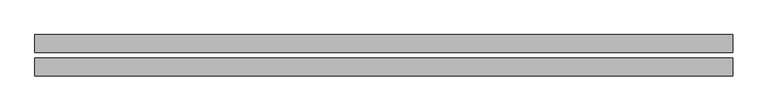
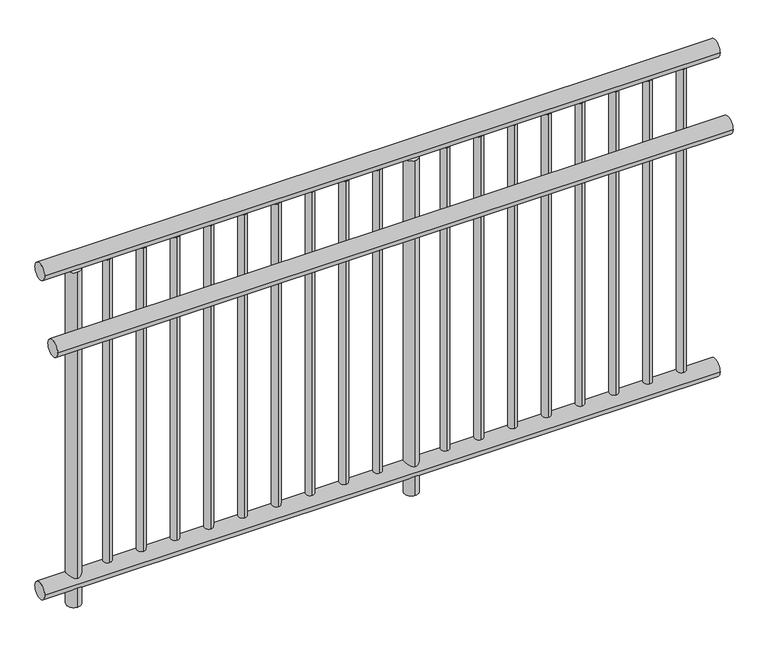
"""IFC4 building model written with IfcOpenShell, lengths in millimetres: railing geometry."""

import ifcopenshell
import ifcopenshell.guid

model = None  # the IFC model being written
_history = None  # IfcOwnerHistory: only IFC2X3 demands one
_inside = {}  # id of a spatial element -> (the spatial element, [elements in it])
_under = {}  # id of a project, library or spatial element -> (it, [spatial elements below it])
_declared = {}  # id of a project -> (the project, [libraries it declares])
_typed = {}  # id of a type object -> (the type object, [elements of that type])
_made_of = {}  # id of a material, layer set ... -> (it, [elements and type objects made of it])


def new_model(schema):
    """Start an empty IFC model of exactly this schema.

    Asked for "IFC4X3", IfcOpenShell would pick the latest addendum, in which some entities
    have other attributes; the version numbers below select the first issue.
    IFC2X3 requires an IfcOwnerHistory on every rooted entity: one is made here for all.
    """
    global model, _history
    if schema == "IFC4X3":
        model = ifcopenshell.file(schema_version=(4, 3, 0, 0))
    else:
        model = ifcopenshell.file(schema=schema)
    _inside.clear()
    _under.clear()
    _declared.clear()
    _typed.clear()
    _made_of.clear()
    _history = None
    if model.schema == "IFC2X3":
        org = make("IfcOrganization", Name="unknown")
        user = make(
            "IfcPersonAndOrganization",
            ThePerson=make("IfcPerson", FamilyName="unknown"),
            TheOrganization=org,
        )
        app = make(
            "IfcApplication",
            ApplicationDeveloper=org,
            Version="unknown",
            ApplicationFullName="unknown",
            ApplicationIdentifier="unknown",
        )
        _history = make(
            "IfcOwnerHistory",
            OwningUser=user,
            OwningApplication=app,
            ChangeAction="ADDED",
            CreationDate=0,
        )
    return model


def make(cls, **values):
    """One entity of the class cls with the attributes given. An attribute that is None is left unset."""
    return model.create_entity(
        cls, **{name: value for name, value in values.items() if value is not None}
    )


def rooted(cls, **values):
    """An entity with a GlobalId (a new one), such as an element, a storey or a relation."""
    return make(cls, GlobalId=ifcopenshell.guid.new(), OwnerHistory=_history, **values)


def si_unit(unit_type, name, prefix=None):
    """IfcSIUnit, for example si_unit("LENGTHUNIT", "METRE", prefix="MILLI")."""
    return make("IfcSIUnit", UnitType=unit_type, Prefix=prefix, Name=name)


def assignment(units):
    """IfcUnitAssignment: the units of a project."""
    return None if units is None else make("IfcUnitAssignment", Units=units)


def point(xyz):
    """IfcCartesianPoint."""
    return None if xyz is None else make("IfcCartesianPoint", Coordinates=xyz)


def direction(xyz):
    """IfcDirection."""
    return None if xyz is None else make("IfcDirection", DirectionRatios=xyz)


def frame(location, z_axis=None, x_axis=None):
    """IfcAxis2Placement3D, a coordinate frame: its origin and axes. An axis left out is left unset."""
    return make(
        "IfcAxis2Placement3D",
        Location=point(location),
        Axis=direction(z_axis),
        RefDirection=direction(x_axis),
    )


def frame_2d(location, x_axis=None):
    """IfcAxis2Placement2D, a coordinate frame in the plane: its origin and x axis."""
    return make(
        "IfcAxis2Placement2D", Location=point(location), RefDirection=direction(x_axis)
    )


def origin():
    """The frame at (0, 0, 0) with its axes left unset."""
    return frame((0.0, 0.0, 0.0))


def origin_with_axes():
    """The frame at (0, 0, 0) with the z axis (0, 0, 1) and the x axis (1, 0, 0) written out."""
    return frame((0.0, 0.0, 0.0), z_axis=(0.0, 0.0, 1.0), x_axis=(1.0, 0.0, 0.0))


def place(relative_to, where):
    """IfcLocalPlacement: puts the frame where relative to a parent placement (None: the world)."""
    return make(
        "IfcLocalPlacement", PlacementRelTo=relative_to, RelativePlacement=where
    )


def context(
    kind, dimensions, precision=None, world=None, true_north=None, identifier=None
):
    """IfcGeometricRepresentationContext, for example the 3D "Model" context."""
    return make(
        "IfcGeometricRepresentationContext",
        ContextIdentifier=identifier,
        ContextType=kind,
        CoordinateSpaceDimension=dimensions,
        Precision=precision,
        WorldCoordinateSystem=world,
        TrueNorth=true_north,
    )


def project(units=None, contexts=None):
    """IfcProject with its units and contexts."""
    return rooted(
        "IfcProject",
        Name="project",
        RepresentationContexts=contexts,
        UnitsInContext=assignment(units),
    )


def spatial(cls, under=None, at=None, **own):
    """A site, building, storey or space (cls), placed at a placement, below another one or the project."""
    s = rooted(cls, ObjectPlacement=at, **own)
    if under is not None:
        _under.setdefault(under.id(), (under, []))[1].append(s)
    return s


def circle_curve(where, radius):
    """IfcCircle in the frame where."""
    return make("IfcCircle", Position=where, Radius=radius)


def trimmed(basis, trim1, trim2, sense, master):
    """IfcTrimmedCurve: the piece of a basis curve between two trims."""
    return make(
        "IfcTrimmedCurve",
        BasisCurve=basis,
        Trim1=trim1,
        Trim2=trim2,
        SenseAgreement=sense,
        MasterRepresentation=master,
    )


def segment(curve, same_sense, transition):
    """IfcCompositeCurveSegment."""
    return make(
        "IfcCompositeCurveSegment",
        Transition=transition,
        SameSense=same_sense,
        ParentCurve=curve,
    )


def composite_curve(segments, self_intersect=None):
    """IfcCompositeCurve: segments joined end to end."""
    return make("IfcCompositeCurve", Segments=segments, SelfIntersect=self_intersect)


def outline(outer, holes=None, kind="AREA"):
    """IfcArbitraryClosedProfileDef: a profile drawn as a closed curve; with holes, ...WithVoids."""
    if holes is None:
        return make("IfcArbitraryClosedProfileDef", ProfileType=kind, OuterCurve=outer)
    return make(
        "IfcArbitraryProfileDefWithVoids",
        ProfileType=kind,
        OuterCurve=outer,
        InnerCurves=holes,
    )


def extrude(swept, where, along, depth):
    """IfcExtrudedAreaSolid: the profile swept, set in the frame where, extruded along a direction by depth."""
    return make(
        "IfcExtrudedAreaSolid",
        SweptArea=swept,
        Position=where,
        ExtrudedDirection=direction(along),
        Depth=depth,
    )


def shape(context_of_items, identifier, shape_type, items):
    """IfcShapeRepresentation: the items that make up one representation, for example the "Body"."""
    return make(
        "IfcShapeRepresentation",
        ContextOfItems=context_of_items,
        RepresentationIdentifier=identifier,
        RepresentationType=shape_type,
        Items=items,
    )


def source(mapping_origin, context_of_items, identifier, shape_type, items):
    """IfcRepresentationMap: a shape defined once, which mapped items show again and again."""
    return make(
        "IfcRepresentationMap",
        MappingOrigin=mapping_origin,
        MappedRepresentation=shape(context_of_items, identifier, shape_type, items),
    )


def transform(
    local_origin,
    x_axis=None,
    y_axis=None,
    z_axis=None,
    scale=None,
    scale2=None,
    scale3=None,
    uniform=True,
):
    """IfcCartesianTransformationOperator3D, or its non-uniform kind. x_axis, y_axis, z_axis: its Axis1, 2, 3."""
    if uniform:
        return make(
            "IfcCartesianTransformationOperator3D",
            Axis1=direction(x_axis),
            Axis2=direction(y_axis),
            LocalOrigin=point(local_origin),
            Scale=scale,
            Axis3=direction(z_axis),
        )
    return make(
        "IfcCartesianTransformationOperator3DnonUniform",
        Axis1=direction(x_axis),
        Axis2=direction(y_axis),
        LocalOrigin=point(local_origin),
        Scale=scale,
        Axis3=direction(z_axis),
        Scale2=scale2,
        Scale3=scale3,
    )


def mapped(mapping_source, mapping_target):
    """IfcMappedItem: shows the shape of a source again, moved by a transform."""
    return make(
        "IfcMappedItem", MappingSource=mapping_source, MappingTarget=mapping_target
    )


def made_of(thing, what):
    """Note that an element or type object is made of a material, layer set ...; save() writes the relation."""
    if what is not None:
        _made_of.setdefault(what.id(), (what, []))[1].append(thing)
    return thing


def element(
    cls,
    number,
    at=None,
    inside=None,
    cuts=None,
    type_object=None,
    material=None,
    context=None,
    identifier="Body",
    shape_type=None,
    held_by="IfcProductDefinitionShape",
    body=None,
    shapes=None,
    **own,
):
    """One element of the class cls, such as IfcWall. Its Tag is "e" and its number.

    at: its placement. inside: the storey or other place that contains it. cuts: it is an
    opening in that element (IfcRelVoidsElement). A single representation is given by context,
    identifier, shape_type and body (its items); several are given by shapes. held_by: the class
    of the entity that holds the representations. save() writes the other relations.
    """
    e = rooted(cls, Tag="e%d" % number, ObjectPlacement=at, **own)
    if body is not None:
        shapes = [shape(context, identifier, shape_type, body)]
    if shapes is not None:
        e.Representation = make(held_by, Representations=shapes)
    if inside is not None:
        _inside.setdefault(inside.id(), (inside, []))[1].append(e)
    if cuts is not None:
        rooted(
            "IfcRelVoidsElement", RelatingBuildingElement=cuts, RelatedOpeningElement=e
        )
    if type_object is not None:
        _typed.setdefault(type_object.id(), (type_object, []))[1].append(e)
    return made_of(e, material)


def aggregate(whole, parts):
    """IfcRelAggregates: a whole, such as a stair, and the parts it consists of."""
    return rooted("IfcRelAggregates", RelatingObject=whole, RelatedObjects=parts)


def save(model, path):
    """Write the relations noted so far, then the file.

    IfcRelAggregates (storeys below a building ...), IfcRelContainedInSpatialStructure (elements
    in a storey), IfcRelDefinesByType, IfcRelAssociatesMaterial and IfcRelDeclares: one each for
    every whole, place, type object, material and project.
    """
    for whole, parts in _under.values():
        aggregate(whole, parts)
    for where, things in _inside.values():
        rooted(
            "IfcRelContainedInSpatialStructure",
            RelatedElements=things,
            RelatingStructure=where,
        )
    for kind, things in _typed.values():
        rooted("IfcRelDefinesByType", RelatedObjects=things, RelatingType=kind)
    for what, things in _made_of.values():
        rooted("IfcRelAssociatesMaterial", RelatedObjects=things, RelatingMaterial=what)
    for by, libraries in _declared.values():
        rooted("IfcRelDeclares", RelatingContext=by, RelatedDefinitions=libraries)
    model.write(path)


def railing_eefe8ac2(model_context):
    return source(origin(), model_context, "Body", "SweptSolid", [
        extrude(outline(composite_curve([segment(trimmed(circle_curve(frame_2d((29848.1400611, 1074.6)), 25.4), [point((29873.5400611, 1074.6))], [point((29822.7400611, 1074.6))], False, "CARTESIAN"), True, "CONTINUOUS"), segment(trimmed(circle_curve(frame_2d((29848.1400611, 1074.6)), 25.4), [point((29822.7400611, 1074.6))], [point((29873.5400611, 1074.6))], False, "CARTESIAN"), True, "CONTINUOUS")], self_intersect=False)), frame((9666.6129185, 0.0, 0.0), z_axis=(1.0, 0.0, 0.0), x_axis=(0.0, 1.0, 0.0)), (0.0, 0.0, 1.0), 2000.0),
        extrude(outline(composite_curve([segment(trimmed(circle_curve(frame_2d((29781.1400611, 874.6)), 25.4), [point((29806.5400611, 874.6))], [point((29755.7400611, 874.6))], False, "CARTESIAN"), True, "CONTINUOUS"), segment(trimmed(circle_curve(frame_2d((29781.1400611, 874.6)), 25.4), [point((29755.7400611, 874.6))], [point((29806.5400611, 874.6))], False, "CARTESIAN"), True, "CONTINUOUS")], self_intersect=False)), frame((9666.6129185, 0.0, 0.0), z_axis=(1.0, 0.0, 0.0), x_axis=(0.0, 1.0, 0.0)), (0.0, 0.0, 1.0), 2000.0),
        extrude(outline(composite_curve([segment(trimmed(circle_curve(frame_2d((29848.1400611, 74.6)), 25.4), [point((29873.5400611, 74.6))], [point((29822.7400611, 74.6))], False, "CARTESIAN"), True, "CONTINUOUS"), segment(trimmed(circle_curve(frame_2d((29848.1400611, 74.6)), 25.4), [point((29822.7400611, 74.6))], [point((29873.5400611, 74.6))], False, "CARTESIAN"), True, "CONTINUOUS")], self_intersect=False)), frame((9666.6129185, 0.0, 0.0), z_axis=(1.0, 0.0, 0.0), x_axis=(0.0, 1.0, 0.0)), (0.0, 0.0, 1.0), 2000.0),
        extrude(outline(composite_curve([segment(trimmed(circle_curve(frame_2d((11566.6129185, 29848.1400611)), 12.5), [point((11566.6129185, 29860.6400611))], [point((11566.6129185, 29835.6400611))], False, "CARTESIAN"), True, "CONTINUOUS"), segment(trimmed(circle_curve(frame_2d((11566.6129185, 29848.1400611)), 12.5), [point((11566.6129185, 29835.6400611))], [point((11566.6129185, 29860.6400611))], False, "CARTESIAN"), True, "CONTINUOUS")], self_intersect=False)), frame((0.0, 0.0, 100.0), z_axis=(0.0, 0.0, 1.0), x_axis=(1.0, 0.0, 0.0)), (0.0, 0.0, 1.0), 949.2),
        extrude(outline(composite_curve([segment(trimmed(circle_curve(frame_2d((11466.6129185, 29848.1400611)), 12.5), [point((11466.6129185, 29860.6400611))], [point((11466.6129185, 29835.6400611))], False, "CARTESIAN"), True, "CONTINUOUS"), segment(trimmed(circle_curve(frame_2d((11466.6129185, 29848.1400611)), 12.5), [point((11466.6129185, 29835.6400611))], [point((11466.6129185, 29860.6400611))], False, "CARTESIAN"), True, "CONTINUOUS")], self_intersect=False)), frame((0.0, 0.0, 100.0), z_axis=(0.0, 0.0, 1.0), x_axis=(1.0, 0.0, 0.0)), (0.0, 0.0, 1.0), 949.2),
        extrude(outline(composite_curve([segment(trimmed(circle_curve(frame_2d((11366.6129185, 29848.1400611)), 12.5), [point((11366.6129185, 29860.6400611))], [point((11366.6129185, 29835.6400611))], False, "CARTESIAN"), True, "CONTINUOUS"), segment(trimmed(circle_curve(frame_2d((11366.6129185, 29848.1400611)), 12.5), [point((11366.6129185, 29835.6400611))], [point((11366.6129185, 29860.6400611))], False, "CARTESIAN"), True, "CONTINUOUS")], self_intersect=False)), frame((0.0, 0.0, 100.0), z_axis=(0.0, 0.0, 1.0), x_axis=(1.0, 0.0, 0.0)), (0.0, 0.0, 1.0), 949.2),
        extrude(outline(composite_curve([segment(trimmed(circle_curve(frame_2d((11266.6129185, 29848.1400611)), 12.5), [point((11266.6129185, 29860.6400611))], [point((11266.6129185, 29835.6400611))], False, "CARTESIAN"), True, "CONTINUOUS"), segment(trimmed(circle_curve(frame_2d((11266.6129185, 29848.1400611)), 12.5), [point((11266.6129185, 29835.6400611))], [point((11266.6129185, 29860.6400611))], False, "CARTESIAN"), True, "CONTINUOUS")], self_intersect=False)), frame((0.0, 0.0, 100.0), z_axis=(0.0, 0.0, 1.0), x_axis=(1.0, 0.0, 0.0)), (0.0, 0.0, 1.0), 949.2),
        extrude(outline(composite_curve([segment(trimmed(circle_curve(frame_2d((11166.6129185, 29848.1400611)), 12.5), [point((11166.6129185, 29860.6400611))], [point((11166.6129185, 29835.6400611))], False, "CARTESIAN"), True, "CONTINUOUS"), segment(trimmed(circle_curve(frame_2d((11166.6129185, 29848.1400611)), 12.5), [point((11166.6129185, 29835.6400611))], [point((11166.6129185, 29860.6400611))], False, "CARTESIAN"), True, "CONTINUOUS")], self_intersect=False)), frame((0.0, 0.0, 100.0), z_axis=(0.0, 0.0, 1.0), x_axis=(1.0, 0.0, 0.0)), (0.0, 0.0, 1.0), 949.2),
        extrude(outline(composite_curve([segment(trimmed(circle_curve(frame_2d((11066.6129185, 29848.1400611)), 12.5), [point((11066.6129185, 29860.6400611))], [point((11066.6129185, 29835.6400611))], False, "CARTESIAN"), True, "CONTINUOUS"), segment(trimmed(circle_curve(frame_2d((11066.6129185, 29848.1400611)), 12.5), [point((11066.6129185, 29835.6400611))], [point((11066.6129185, 29860.6400611))], False, "CARTESIAN"), True, "CONTINUOUS")], self_intersect=False)), frame((0.0, 0.0, 100.0), z_axis=(0.0, 0.0, 1.0), x_axis=(1.0, 0.0, 0.0)), (0.0, 0.0, 1.0), 949.2),
        extrude(outline(composite_curve([segment(trimmed(circle_curve(frame_2d((10966.6129185, 29848.1400611)), 12.5), [point((10966.6129185, 29860.6400611))], [point((10966.6129185, 29835.6400611))], False, "CARTESIAN"), True, "CONTINUOUS"), segment(trimmed(circle_curve(frame_2d((10966.6129185, 29848.1400611)), 12.5), [point((10966.6129185, 29835.6400611))], [point((10966.6129185, 29860.6400611))], False, "CARTESIAN"), True, "CONTINUOUS")], self_intersect=False)), frame((0.0, 0.0, 100.0), z_axis=(0.0, 0.0, 1.0), x_axis=(1.0, 0.0, 0.0)), (0.0, 0.0, 1.0), 949.2),
        extrude(outline(composite_curve([segment(trimmed(circle_curve(frame_2d((10866.6129185, 29848.1400611)), 12.5), [point((10866.6129185, 29860.6400611))], [point((10866.6129185, 29835.6400611))], False, "CARTESIAN"), True, "CONTINUOUS"), segment(trimmed(circle_curve(frame_2d((10866.6129185, 29848.1400611)), 12.5), [point((10866.6129185, 29835.6400611))], [point((10866.6129185, 29860.6400611))], False, "CARTESIAN"), True, "CONTINUOUS")], self_intersect=False)), frame((0.0, 0.0, 100.0), z_axis=(0.0, 0.0, 1.0), x_axis=(1.0, 0.0, 0.0)), (0.0, 0.0, 1.0), 949.2),
        extrude(outline(composite_curve([segment(trimmed(circle_curve(frame_2d((10766.6129185, 29848.1400611)), 21.0), [point((10766.6129185, 29869.1400611))], [point((10766.6129185, 29827.1400611))], False, "CARTESIAN"), True, "CONTINUOUS"), segment(trimmed(circle_curve(frame_2d((10766.6129185, 29848.1400611)), 21.0), [point((10766.6129185, 29827.1400611))], [point((10766.6129185, 29869.1400611))], False, "CARTESIAN"), True, "CONTINUOUS")], self_intersect=False)), origin_with_axes(), (0.0, 0.0, 1.0), 1049.2),
        extrude(outline(composite_curve([segment(trimmed(circle_curve(frame_2d((10666.6129185, 29848.1400611)), 12.5), [point((10666.6129185, 29860.6400611))], [point((10666.6129185, 29835.6400611))], False, "CARTESIAN"), True, "CONTINUOUS"), segment(trimmed(circle_curve(frame_2d((10666.6129185, 29848.1400611)), 12.5), [point((10666.6129185, 29835.6400611))], [point((10666.6129185, 29860.6400611))], False, "CARTESIAN"), True, "CONTINUOUS")], self_intersect=False)), frame((0.0, 0.0, 100.0), z_axis=(0.0, 0.0, 1.0), x_axis=(1.0, 0.0, 0.0)), (0.0, 0.0, 1.0), 949.2),
        extrude(outline(composite_curve([segment(trimmed(circle_curve(frame_2d((10566.6129185, 29848.1400611)), 12.5), [point((10566.6129185, 29860.6400611))], [point((10566.6129185, 29835.6400611))], False, "CARTESIAN"), True, "CONTINUOUS"), segment(trimmed(circle_curve(frame_2d((10566.6129185, 29848.1400611)), 12.5), [point((10566.6129185, 29835.6400611))], [point((10566.6129185, 29860.6400611))], False, "CARTESIAN"), True, "CONTINUOUS")], self_intersect=False)), frame((0.0, 0.0, 100.0), z_axis=(0.0, 0.0, 1.0), x_axis=(1.0, 0.0, 0.0)), (0.0, 0.0, 1.0), 949.2),
        extrude(outline(composite_curve([segment(trimmed(circle_curve(frame_2d((10466.6129185, 29848.1400611)), 12.5), [point((10466.6129185, 29860.6400611))], [point((10466.6129185, 29835.6400611))], False, "CARTESIAN"), True, "CONTINUOUS"), segment(trimmed(circle_curve(frame_2d((10466.6129185, 29848.1400611)), 12.5), [point((10466.6129185, 29835.6400611))], [point((10466.6129185, 29860.6400611))], False, "CARTESIAN"), True, "CONTINUOUS")], self_intersect=False)), frame((0.0, 0.0, 100.0), z_axis=(0.0, 0.0, 1.0), x_axis=(1.0, 0.0, 0.0)), (0.0, 0.0, 1.0), 949.2),
        extrude(outline(composite_curve([segment(trimmed(circle_curve(frame_2d((10366.6129185, 29848.1400611)), 12.5), [point((10366.6129185, 29860.6400611))], [point((10366.6129185, 29835.6400611))], False, "CARTESIAN"), True, "CONTINUOUS"), segment(trimmed(circle_curve(frame_2d((10366.6129185, 29848.1400611)), 12.5), [point((10366.6129185, 29835.6400611))], [point((10366.6129185, 29860.6400611))], False, "CARTESIAN"), True, "CONTINUOUS")], self_intersect=False)), frame((0.0, 0.0, 100.0), z_axis=(0.0, 0.0, 1.0), x_axis=(1.0, 0.0, 0.0)), (0.0, 0.0, 1.0), 949.2),
        extrude(outline(composite_curve([segment(trimmed(circle_curve(frame_2d((10266.6129185, 29848.1400611)), 12.5), [point((10266.6129185, 29860.6400611))], [point((10266.6129185, 29835.6400611))], False, "CARTESIAN"), True, "CONTINUOUS"), segment(trimmed(circle_curve(frame_2d((10266.6129185, 29848.1400611)), 12.5), [point((10266.6129185, 29835.6400611))], [point((10266.6129185, 29860.6400611))], False, "CARTESIAN"), True, "CONTINUOUS")], self_intersect=False)), frame((0.0, 0.0, 100.0), z_axis=(0.0, 0.0, 1.0), x_axis=(1.0, 0.0, 0.0)), (0.0, 0.0, 1.0), 949.2),
        extrude(outline(composite_curve([segment(trimmed(circle_curve(frame_2d((10166.6129185, 29848.1400611)), 12.5), [point((10166.6129185, 29860.6400611))], [point((10166.6129185, 29835.6400611))], False, "CARTESIAN"), True, "CONTINUOUS"), segment(trimmed(circle_curve(frame_2d((10166.6129185, 29848.1400611)), 12.5), [point((10166.6129185, 29835.6400611))], [point((10166.6129185, 29860.6400611))], False, "CARTESIAN"), True, "CONTINUOUS")], self_intersect=False)), frame((0.0, 0.0, 100.0), z_axis=(0.0, 0.0, 1.0), x_axis=(1.0, 0.0, 0.0)), (0.0, 0.0, 1.0), 949.2),
        extrude(outline(composite_curve([segment(trimmed(circle_curve(frame_2d((10066.6129185, 29848.1400611)), 12.5), [point((10066.6129185, 29860.6400611))], [point((10066.6129185, 29835.6400611))], False, "CARTESIAN"), True, "CONTINUOUS"), segment(trimmed(circle_curve(frame_2d((10066.6129185, 29848.1400611)), 12.5), [point((10066.6129185, 29835.6400611))], [point((10066.6129185, 29860.6400611))], False, "CARTESIAN"), True, "CONTINUOUS")], self_intersect=False)), frame((0.0, 0.0, 100.0), z_axis=(0.0, 0.0, 1.0), x_axis=(1.0, 0.0, 0.0)), (0.0, 0.0, 1.0), 949.2),
        extrude(outline(composite_curve([segment(trimmed(circle_curve(frame_2d((9966.6129185, 29848.1400611)), 12.5), [point((9966.6129185, 29860.6400611))], [point((9966.6129185, 29835.6400611))], False, "CARTESIAN"), True, "CONTINUOUS"), segment(trimmed(circle_curve(frame_2d((9966.6129185, 29848.1400611)), 12.5), [point((9966.6129185, 29835.6400611))], [point((9966.6129185, 29860.6400611))], False, "CARTESIAN"), True, "CONTINUOUS")], self_intersect=False)), frame((0.0, 0.0, 100.0), z_axis=(0.0, 0.0, 1.0), x_axis=(1.0, 0.0, 0.0)), (0.0, 0.0, 1.0), 949.2),
        extrude(outline(composite_curve([segment(trimmed(circle_curve(frame_2d((9866.6129185, 29848.1400611)), 12.5), [point((9866.6129185, 29860.6400611))], [point((9866.6129185, 29835.6400611))], False, "CARTESIAN"), True, "CONTINUOUS"), segment(trimmed(circle_curve(frame_2d((9866.6129185, 29848.1400611)), 12.5), [point((9866.6129185, 29835.6400611))], [point((9866.6129185, 29860.6400611))], False, "CARTESIAN"), True, "CONTINUOUS")], self_intersect=False)), frame((0.0, 0.0, 100.0), z_axis=(0.0, 0.0, 1.0), x_axis=(1.0, 0.0, 0.0)), (0.0, 0.0, 1.0), 949.2),
        extrude(outline(composite_curve([segment(trimmed(circle_curve(frame_2d((9766.6129185, 29848.1400611)), 21.0), [point((9766.6129185, 29869.1400611))], [point((9766.6129185, 29827.1400611))], False, "CARTESIAN"), True, "CONTINUOUS"), segment(trimmed(circle_curve(frame_2d((9766.6129185, 29848.1400611)), 21.0), [point((9766.6129185, 29827.1400611))], [point((9766.6129185, 29869.1400611))], False, "CARTESIAN"), True, "CONTINUOUS")], self_intersect=False)), origin_with_axes(), (0.0, 0.0, 1.0), 1049.2),
    ])


if __name__ == "__main__":
    model = new_model("IFC4")
    model_context = context("Model", 3, world=origin())
    ifc_project = project(units=[si_unit("LENGTHUNIT", "METRE", prefix="MILLI")], contexts=[model_context])
    site = spatial("IfcSite", under=ifc_project)
    building = spatial("IfcBuilding", under=site)
    placement = place(None, origin())
    railing_shape = railing_eefe8ac2(model_context)
    element("IfcRailing", 1, at=placement, inside=building, context=model_context, shape_type="MappedRepresentation", body=[
        mapped(railing_shape, transform((0.0, 0.0, 0.0), x_axis=(1.0, 0.0, 0.0), y_axis=(0.0, 1.0, 0.0), z_axis=(0.0, 0.0, 1.0))),
    ])
    save(model, "model.ifc")

# Revit data of these elements
# Element 1 (IfcRailing)
#   Materials on its faces: "Ferro - Pintura Esmalte"
# Materials
#   "Ferro - Pintura Esmalte": class "Pintura", colour RGB 255 255 255, transparency 0, Cost = 0
